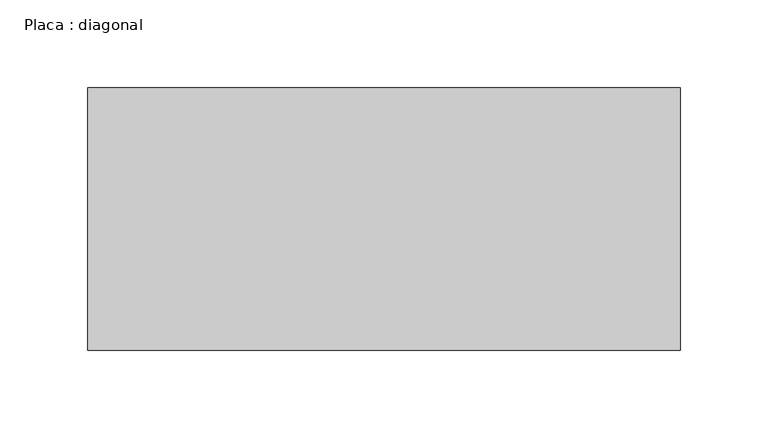
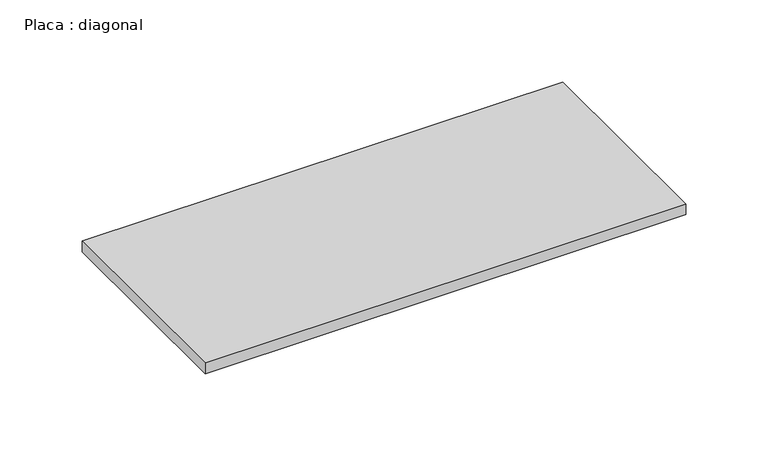
"""IFC4 building model written with IfcOpenShell, lengths in millimetres: beam geometry, Placa : diagonal."""

from ifc_helpers import new_model, si_unit, frame, origin, place, context, project, spatial, polyline, outline, extrude, source, transform, mapped, element, save


def placa_diagonal_99230a8a(model_context):
    return source(origin(), model_context, "Body", "SweptSolid", [
        extrude(outline(polyline([(169.7267346, 75.0), (169.7267346, -75.0), (-168.8798643, -75.0), (-168.8798643, 75.0), (169.7267346, 75.0)])), frame((0.0, 0.0, -4.0), z_axis=(0.0, 0.0, 1.0), x_axis=(1.0, 0.0, 0.0)), (0.0, 0.0, 1.0), 8.0),
    ])


if __name__ == "__main__":
    model = new_model("IFC4")
    model_context = context("Model", 3, world=origin())
    ifc_project = project(units=[si_unit("LENGTHUNIT", "METRE", prefix="MILLI")], contexts=[model_context])
    site = spatial("IfcSite", under=ifc_project)
    building = spatial("IfcBuilding", under=site)
    placement = place(None, origin())
    placa_diagonal_shape = placa_diagonal_99230a8a(model_context)
    element("IfcBeam", 1, ObjectType="Placa : diagonal", at=placement, inside=building, context=model_context, shape_type="MappedRepresentation", body=[
        mapped(placa_diagonal_shape, transform((0.0, 0.0, 0.0), x_axis=(1.0, 0.0, 0.0), y_axis=(0.0, 1.0, 0.0), z_axis=(0.0, 0.0, 1.0))),
    ])
    save(model, "model.ifc")

# Revit data of these elements
# Type "Placa : diagonal"
#   W = 0
#   Length [instance default] = 1.50 m
#   b = 0.15 m
#   d = 0.008 m
#   A = 0 m²
#   Structural Material [instance default] = Aço, 45-345
# Element 1 (IfcBeam, "Placa : diagonal")
#   Materials on its faces: "Aço, 45-345"
# Materials
#   "Aço, 45-345": class "Metal", colour RGB 247 247 247, transparency 0, Description = "Aço 345 MPa", Cost = 0
